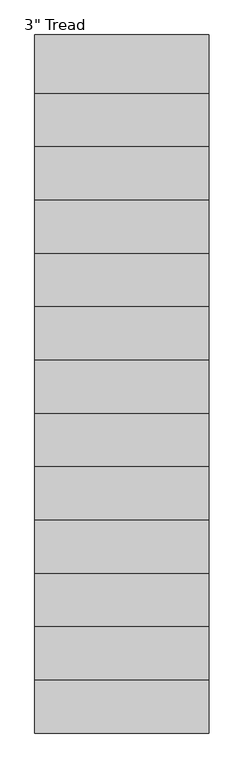
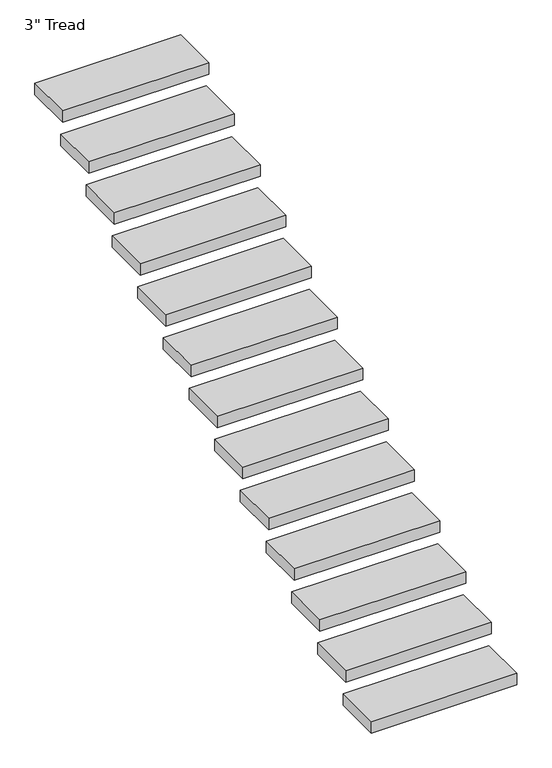
"""IFC4 building model written with IfcOpenShell, lengths in millimetres: stair flight geometry."""

from ifc_helpers import new_model, si_unit, frame, origin, place, context, project, spatial, polyline, outline, extrude, source, transform, mapped, element, save


def stair_flight_4ee9cd7f(model_context):
    return source(origin(), model_context, "Body", "SweptSolid", [
        extrude(outline(polyline([(32168.366427, 31238.5118167), (33082.766427, 31238.5118167), (33082.766427, 30933.7118167), (32168.366427, 30933.7118167), (32168.366427, 31238.5118167)])), frame((0.0, 0.0, 264131.425), z_axis=(0.0, 0.0, 1.0), x_axis=(1.0, 0.0, 0.0)), (0.0, 0.0, 1.0), 76.2),
        extrude(outline(polyline([(32168.366427, 31517.9118167), (33082.766427, 31517.9118167), (33082.766427, 31213.1118167), (32168.366427, 31213.1118167), (32168.366427, 31517.9118167)])), frame((0.0, 0.0, 264299.7), z_axis=(0.0, 0.0, 1.0), x_axis=(1.0, 0.0, 0.0)), (0.0, 0.0, 1.0), 76.2),
        extrude(outline(polyline([(32168.366427, 31797.3118167), (33082.766427, 31797.3118167), (33082.766427, 31492.5118167), (32168.366427, 31492.5118167), (32168.366427, 31797.3118167)])), frame((0.0, 0.0, 264467.975), z_axis=(0.0, 0.0, 1.0), x_axis=(1.0, 0.0, 0.0)), (0.0, 0.0, 1.0), 76.2),
        extrude(outline(polyline([(32168.366427, 32076.7118167), (33082.766427, 32076.7118167), (33082.766427, 31771.9118167), (32168.366427, 31771.9118167), (32168.366427, 32076.7118167)])), frame((0.0, 0.0, 264636.25), z_axis=(0.0, 0.0, 1.0), x_axis=(1.0, 0.0, 0.0)), (0.0, 0.0, 1.0), 76.2),
        extrude(outline(polyline([(32168.366427, 32356.1118167), (33082.766427, 32356.1118167), (33082.766427, 32051.3118167), (32168.366427, 32051.3118167), (32168.366427, 32356.1118167)])), frame((0.0, 0.0, 264804.525), z_axis=(0.0, 0.0, 1.0), x_axis=(1.0, 0.0, 0.0)), (0.0, 0.0, 1.0), 76.2),
        extrude(outline(polyline([(32168.366427, 32635.5118167), (33082.766427, 32635.5118167), (33082.766427, 32330.7118167), (32168.366427, 32330.7118167), (32168.366427, 32635.5118167)])), frame((0.0, 0.0, 264972.8), z_axis=(0.0, 0.0, 1.0), x_axis=(1.0, 0.0, 0.0)), (0.0, 0.0, 1.0), 76.2),
        extrude(outline(polyline([(32168.366427, 32914.9118167), (33082.766427, 32914.9118167), (33082.766427, 32610.1118167), (32168.366427, 32610.1118167), (32168.366427, 32914.9118167)])), frame((0.0, 0.0, 265141.075), z_axis=(0.0, 0.0, 1.0), x_axis=(1.0, 0.0, 0.0)), (0.0, 0.0, 1.0), 76.2),
        extrude(outline(polyline([(32168.366427, 33194.3118167), (33082.766427, 33194.3118167), (33082.766427, 32889.5118167), (32168.366427, 32889.5118167), (32168.366427, 33194.3118167)])), frame((0.0, 0.0, 265309.35), z_axis=(0.0, 0.0, 1.0), x_axis=(1.0, 0.0, 0.0)), (0.0, 0.0, 1.0), 76.2),
        extrude(outline(polyline([(32168.366427, 33473.7118167), (33082.766427, 33473.7118167), (33082.766427, 33168.9118167), (32168.366427, 33168.9118167), (32168.366427, 33473.7118167)])), frame((0.0, 0.0, 265477.625), z_axis=(0.0, 0.0, 1.0), x_axis=(1.0, 0.0, 0.0)), (0.0, 0.0, 1.0), 76.2),
        extrude(outline(polyline([(32168.366427, 33753.1118167), (33082.766427, 33753.1118167), (33082.766427, 33448.3118167), (32168.366427, 33448.3118167), (32168.366427, 33753.1118167)])), frame((0.0, 0.0, 265645.9), z_axis=(0.0, 0.0, 1.0), x_axis=(1.0, 0.0, 0.0)), (0.0, 0.0, 1.0), 76.2),
        extrude(outline(polyline([(32168.366427, 34032.5118167), (33082.766427, 34032.5118167), (33082.766427, 33727.7118167), (32168.366427, 33727.7118167), (32168.366427, 34032.5118167)])), frame((0.0, 0.0, 265814.175), z_axis=(0.0, 0.0, 1.0), x_axis=(1.0, 0.0, 0.0)), (0.0, 0.0, 1.0), 76.2),
        extrude(outline(polyline([(32168.366427, 34311.9118167), (33082.766427, 34311.9118167), (33082.766427, 34007.1118167), (32168.366427, 34007.1118167), (32168.366427, 34311.9118167)])), frame((0.0, 0.0, 265982.45), z_axis=(0.0, 0.0, 1.0), x_axis=(1.0, 0.0, 0.0)), (0.0, 0.0, 1.0), 76.2),
        extrude(outline(polyline([(32168.366427, 34591.3118167), (33082.766427, 34591.3118167), (33082.766427, 34286.5118167), (32168.366427, 34286.5118167), (32168.366427, 34591.3118167)])), frame((0.0, 0.0, 266150.725), z_axis=(0.0, 0.0, 1.0), x_axis=(1.0, 0.0, 0.0)), (0.0, 0.0, 1.0), 76.2),
    ])


if __name__ == "__main__":
    model = new_model("IFC4")
    model_context = context("Model", 3, world=origin())
    ifc_project = project(units=[si_unit("LENGTHUNIT", "METRE", prefix="MILLI")], contexts=[model_context])
    site = spatial("IfcSite", under=ifc_project)
    building = spatial("IfcBuilding", under=site)
    placement = place(None, origin())
    stair_flight_shape = stair_flight_4ee9cd7f(model_context)
    element("IfcStairFlight", 1, ObjectType="3\" Tread", at=placement, inside=building, context=model_context, shape_type="MappedRepresentation", body=[
        mapped(stair_flight_shape, transform((0.0, 0.0, 0.0), x_axis=(1.0, 0.0, 0.0), y_axis=(0.0, 1.0, 0.0), z_axis=(0.0, 0.0, 1.0))),
    ])
    save(model, "model.ifc")

# Revit data of these elements
# Element 1 (IfcStairFlight, "3\" Tread")
#   Materials on its faces: "GLULAMS BEAMS\n(PRESSURE TREATED W/ PENTA IN SOLVENT) (EXTERIOR STAIN: PENOFIN VERDE EXT. STAIN - COLOR: CEDAR)"
# Materials
#   "GLULAMS BEAMS\n(PRESSURE TREATED W/ PENTA IN SOLVENT) (EXTERIOR STAIN: PENOFIN VERDE EXT. STAIN - COLOR: CEDAR)": class "Wood", colour RGB 164 134 123, transparency 0, Description = "Pinus Echinata", Cost = 0
